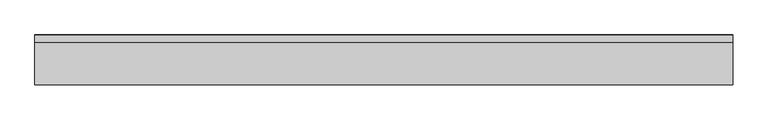
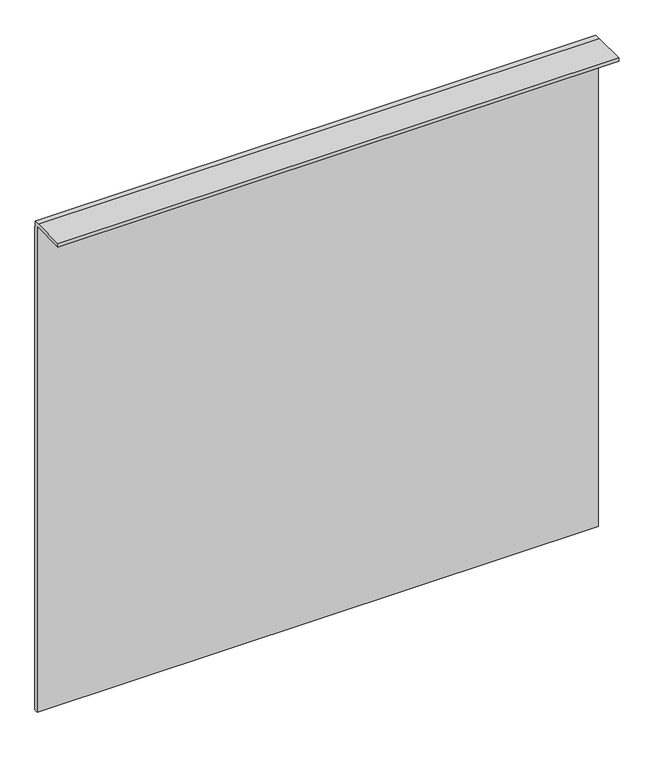
"""IFC4 building model written with IfcOpenShell, lengths in millimetres: proxy geometry, Gypsum018 33917 : Gypsum018 33917."""

from ifc_helpers import new_model, si_unit, frame, origin, place, context, project, spatial, polyline, outline, extrude, source, transform, mapped, element, save


def generic_models_51115563(model_context):
    return source(origin(), model_context, "Body", "SweptSolid", [
        extrude(outline(polyline([(-4483.5542972, 36582.096), (-4497.8425368, 36582.096), (-4497.8425368, 38414.5015625), (-4625.6960524, 38414.5015625), (-4625.6960524, 38427.7398437), (-4505.9874811, 38427.7398437), (-4505.9874811, 38426.4598437), (-4484.8342972, 38426.4598437), (-4484.8342972, 38405.3066598), (-4483.5542972, 38405.3066598), (-4483.5542972, 36582.096)])), frame((12383.0178845, 0.0, 0.0), z_axis=(1.0, 0.0, 0.0), x_axis=(0.0, 1.0, 0.0)), (0.0, 0.0, 1.0), 2000.0),
    ])


if __name__ == "__main__":
    model = new_model("IFC4")
    model_context = context("Model", 3, world=origin())
    ifc_project = project(units=[si_unit("LENGTHUNIT", "METRE", prefix="MILLI")], contexts=[model_context])
    site = spatial("IfcSite", under=ifc_project)
    building = spatial("IfcBuilding", under=site)
    placement = place(None, origin())
    generic_models_shape = generic_models_51115563(model_context)
    element("IfcBuildingElementProxy", 1, Name="Gypsum018 33917 : Gypsum018 33917", ObjectType="Gypsum018 33917 : Gypsum018 33917", at=placement, inside=building, context=model_context, shape_type="MappedRepresentation", body=[
        mapped(generic_models_shape, transform((0.0, 0.0, 0.0), x_axis=(1.0, 0.0, 0.0), y_axis=(0.0, 1.0, 0.0), z_axis=(0.0, 0.0, 1.0))),
    ])
    save(model, "model.ifc")

# Revit data of these elements
# Type "Gypsum018 33917 : Gypsum018 33917"
#   NameOverride = "Gypsum018"
# Element 1 (IfcBuildingElementProxy, "Gypsum018 33917 : Gypsum018 33917")
#   Materials on its faces: "5/8\"  GYPSUM BOARD"
# Materials
#   "5/8\"  GYPSUM BOARD": class "Unassigned", colour RGB 255 255 255, transparency 0, Cost = 0
